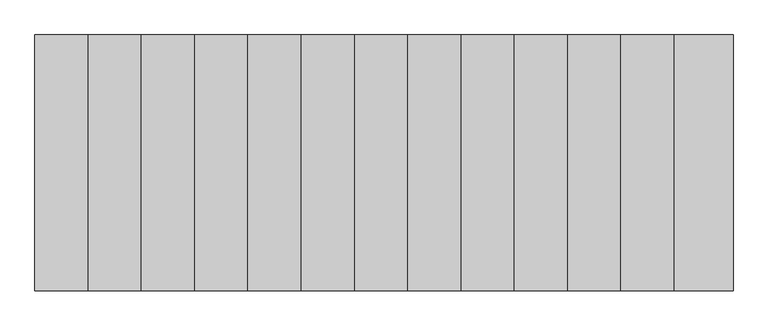
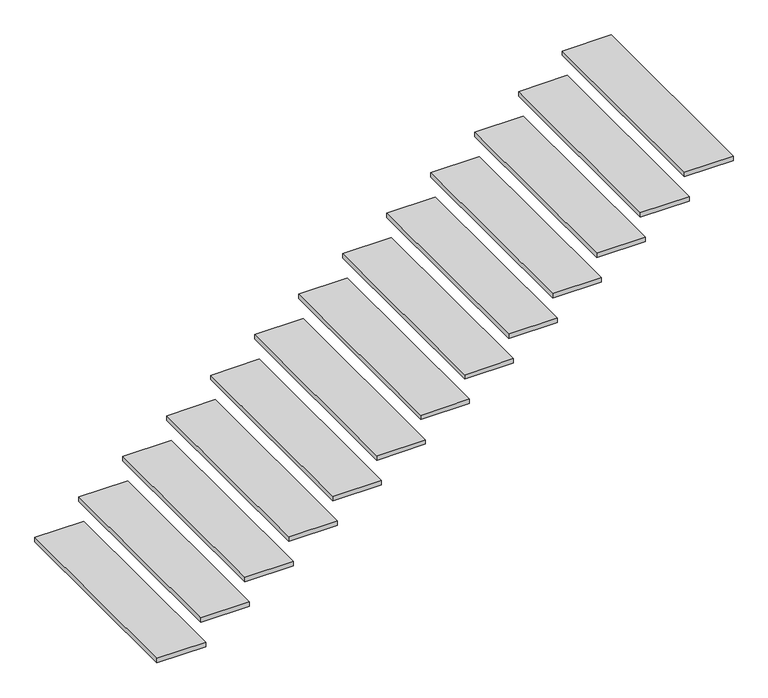
"""IFC4 building model written with IfcOpenShell, lengths in millimetres: stair flight geometry."""

from ifc_helpers import new_model, si_unit, frame, origin, place, context, project, spatial, polyline, outline, extrude, source, transform, mapped, element, save


def stair_flight_12ee3755(model_context):
    return source(origin(), model_context, "Body", "SweptSolid", [
        extrude(outline(polyline([(-7050.3787762, -1414.2822308), (-7050.3787762, -2770.0522873), (-7362.5216334, -2770.0522873), (-7362.5216334, -1414.2822308), (-7050.3787762, -1414.2822308)])), frame((0.0, 0.0, -1423.5714286), z_axis=(0.0, 0.0, 1.0), x_axis=(1.0, 0.0, 0.0)), (0.0, 0.0, 1.0), 30.0),
        extrude(outline(polyline([(-6768.2359191, -1414.2822308), (-6768.2359191, -2770.0522873), (-7080.3787762, -2770.0522873), (-7080.3787762, -1414.2822308), (-6768.2359191, -1414.2822308)])), frame((0.0, 0.0, -1247.1428571), z_axis=(0.0, 0.0, 1.0), x_axis=(1.0, 0.0, 0.0)), (0.0, 0.0, 1.0), 30.0),
        extrude(outline(polyline([(-6486.0930619, -1414.2822308), (-6486.0930619, -2770.0522873), (-6798.2359191, -2770.0522873), (-6798.2359191, -1414.2822308), (-6486.0930619, -1414.2822308)])), frame((0.0, 0.0, -1070.7142857), z_axis=(0.0, 0.0, 1.0), x_axis=(1.0, 0.0, 0.0)), (0.0, 0.0, 1.0), 30.0),
        extrude(outline(polyline([(-6203.9502048, -1414.2822308), (-6203.9502048, -2770.0522873), (-6516.0930619, -2770.0522873), (-6516.0930619, -1414.2822308), (-6203.9502048, -1414.2822308)])), frame((0.0, 0.0, -894.2857143), z_axis=(0.0, 0.0, 1.0), x_axis=(1.0, 0.0, 0.0)), (0.0, 0.0, 1.0), 30.0),
        extrude(outline(polyline([(-5921.8073477, -1414.2822308), (-5921.8073477, -2770.0522873), (-6233.9502048, -2770.0522873), (-6233.9502048, -1414.2822308), (-5921.8073477, -1414.2822308)])), frame((0.0, 0.0, -717.8571429), z_axis=(0.0, 0.0, 1.0), x_axis=(1.0, 0.0, 0.0)), (0.0, 0.0, 1.0), 30.0),
        extrude(outline(polyline([(-5639.6644905, -1414.2822308), (-5639.6644905, -2770.0522873), (-5951.8073477, -2770.0522873), (-5951.8073477, -1414.2822308), (-5639.6644905, -1414.2822308)])), frame((0.0, 0.0, -541.4285714), z_axis=(0.0, 0.0, 1.0), x_axis=(1.0, 0.0, 0.0)), (0.0, 0.0, 1.0), 30.0),
        extrude(outline(polyline([(-5357.5216334, -1414.2822308), (-5357.5216334, -2770.0522873), (-5669.6644905, -2770.0522873), (-5669.6644905, -1414.2822308), (-5357.5216334, -1414.2822308)])), frame((0.0, 0.0, -365.0), z_axis=(0.0, 0.0, 1.0), x_axis=(1.0, 0.0, 0.0)), (0.0, 0.0, 1.0), 30.0),
        extrude(outline(polyline([(-5075.3787762, -1414.2822308), (-5075.3787762, -2770.0522873), (-5387.5216334, -2770.0522873), (-5387.5216334, -1414.2822308), (-5075.3787762, -1414.2822308)])), frame((0.0, 0.0, -188.5714286), z_axis=(0.0, 0.0, 1.0), x_axis=(1.0, 0.0, 0.0)), (0.0, 0.0, 1.0), 30.0),
        extrude(outline(polyline([(-4793.2359191, -1414.2822308), (-4793.2359191, -2770.0522873), (-5105.3787762, -2770.0522873), (-5105.3787762, -1414.2822308), (-4793.2359191, -1414.2822308)])), frame((0.0, 0.0, -12.1428571), z_axis=(0.0, 0.0, 1.0), x_axis=(1.0, 0.0, 0.0)), (0.0, 0.0, 1.0), 30.0),
        extrude(outline(polyline([(-4511.0930619, -1414.2822308), (-4511.0930619, -2770.0522873), (-4823.2359191, -2770.0522873), (-4823.2359191, -1414.2822308), (-4511.0930619, -1414.2822308)])), frame((0.0, 0.0, 164.2857143), z_axis=(0.0, 0.0, 1.0), x_axis=(1.0, 0.0, 0.0)), (0.0, 0.0, 1.0), 30.0),
        extrude(outline(polyline([(-4228.9502048, -1414.2822308), (-4228.9502048, -2770.0522873), (-4541.0930619, -2770.0522873), (-4541.0930619, -1414.2822308), (-4228.9502048, -1414.2822308)])), frame((0.0, 0.0, 340.7142857), z_axis=(0.0, 0.0, 1.0), x_axis=(1.0, 0.0, 0.0)), (0.0, 0.0, 1.0), 30.0),
        extrude(outline(polyline([(-3946.8073477, -1414.2822308), (-3946.8073477, -2770.0522873), (-4258.9502048, -2770.0522873), (-4258.9502048, -1414.2822308), (-3946.8073477, -1414.2822308)])), frame((0.0, 0.0, 517.1428571), z_axis=(0.0, 0.0, 1.0), x_axis=(1.0, 0.0, 0.0)), (0.0, 0.0, 1.0), 30.0),
        extrude(outline(polyline([(-3664.6644905, -1414.2822308), (-3664.6644905, -2770.0522873), (-3976.8073477, -2770.0522873), (-3976.8073477, -1414.2822308), (-3664.6644905, -1414.2822308)])), frame((0.0, 0.0, 693.5714286), z_axis=(0.0, 0.0, 1.0), x_axis=(1.0, 0.0, 0.0)), (0.0, 0.0, 1.0), 30.0),
    ])


if __name__ == "__main__":
    model = new_model("IFC4")
    model_context = context("Model", 3, world=origin())
    ifc_project = project(units=[si_unit("LENGTHUNIT", "METRE", prefix="MILLI")], contexts=[model_context])
    site = spatial("IfcSite", under=ifc_project)
    building = spatial("IfcBuilding", under=site)
    placement = place(None, origin())
    stair_flight_shape = stair_flight_12ee3755(model_context)
    element("IfcStairFlight", 1, at=placement, inside=building, context=model_context, shape_type="MappedRepresentation", body=[
        mapped(stair_flight_shape, transform((0.0, 0.0, 0.0), x_axis=(1.0, 0.0, 0.0), y_axis=(0.0, 1.0, 0.0), z_axis=(0.0, 0.0, 1.0))),
    ])
    save(model, "model.ifc")

# Revit data of these elements
# Element 1 (IfcStairFlight)
#   Materials on its faces: "Stahlbeton - Sichtbeton (2)"
# Materials
#   "Stahlbeton - Sichtbeton (2)": class "Beton", colour RGB 192 192 192, transparency 0, Cost = 0
